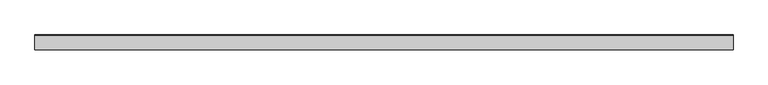
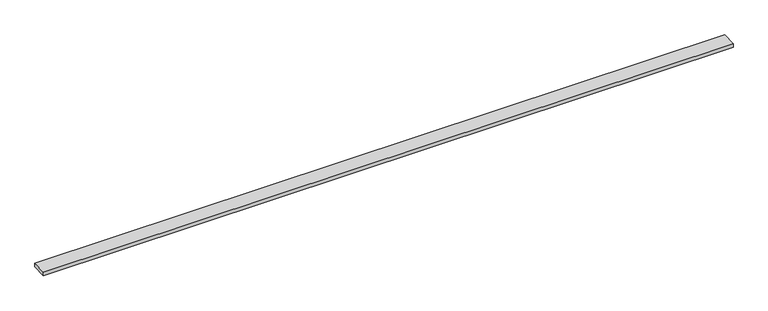
"""IFC4 building model written with IfcOpenShell, lengths in millimetres: proxy geometry, Inner panel:Inner panel:1:Inner panel:1 : Inner panel:Inner panel:300324:2:Inner panel:1:Inner panel:1 : Inner panel:Inner panel:300324:2 : Inner panel:Inner panel:1:Inner panel:1 : Inner panel:Inner panel:300324:300043:9 : Inner panel:Inner panel:1:Inner panel:1 : Inner panel:Inner panel:300324:2:Inner panel:1:Inner panel:1 : Inner panel:Inner panel:300324:2 : Inner panel:Inner panel:1:Inner panel:1 : Inner panel:Inner panel:300324:300043:308120."""

from ifc_helpers import new_model, si_unit, frame, origin, place, context, project, spatial, polyline, outline, extrude, source, transform, mapped, element, save


def generic_models_4ea8c6c7(model_context):
    return source(origin(), model_context, "Body", "SweptSolid", [
        extrude(outline(polyline([(0.0, -102.7190976), (0.0, 0.0), (4876.8, 0.0), (4876.8, -102.7190976), (0.0, -102.7190976)])), frame((596182.8367242, -536656.3145522, 10092.0375334), z_axis=(0.0, -0.04163054471218835, 0.9991330730923517), x_axis=(-1.0, 0.0, 0.0)), (0.0, 0.0, 1.0), 25.4),
    ])


if __name__ == "__main__":
    model = new_model("IFC4")
    model_context = context("Model", 3, world=origin())
    ifc_project = project(units=[si_unit("LENGTHUNIT", "METRE", prefix="MILLI")], contexts=[model_context])
    site = spatial("IfcSite", under=ifc_project)
    building = spatial("IfcBuilding", under=site)
    placement = place(None, origin())
    generic_models_shape = generic_models_4ea8c6c7(model_context)
    element("IfcBuildingElementProxy", 1, Name="Inner panel:Inner panel:1:Inner panel:1 : Inner panel:Inner panel:300324:2:Inner panel:1:Inner panel:1 : Inner panel:Inner panel:300324:2 : Inner panel:Inner panel:1:Inner panel:1 : Inner panel:Inner panel:300324:300043:9 : Inner panel:Inner panel:1:Inner panel:1 : Inner panel:Inner panel:300324:2:Inner panel:1:Inner panel:1 : Inner panel:Inner panel:300324:2 : Inner panel:Inner panel:1:Inner panel:1 : Inner panel:Inner panel:300324:300043:308120", ObjectType="Inner panel:Inner panel:1:Inner panel:1 : Inner panel:Inner panel:300324:2:Inner panel:1:Inner panel:1 : Inner panel:Inner panel:300324:2 : Inner panel:Inner panel:1:Inner panel:1 : Inner panel:Inner panel:300324:300043:9 : Inner panel:Inner panel:1:Inner panel:1 : Inner panel:Inner panel:300324:2:Inner panel:1:Inner panel:1 : Inner panel:Inner panel:300324:2 : Inner panel:Inner panel:1:Inner panel:1 : Inner panel:Inner panel:300324:300043:308120", at=placement, inside=building, context=model_context, shape_type="MappedRepresentation", body=[
        mapped(generic_models_shape, transform((0.0, 0.0, 0.0), x_axis=(1.0, 0.0, 0.0), y_axis=(0.0, 1.0, 0.0), z_axis=(0.0, 0.0, 1.0))),
    ])
    save(model, "model.ifc")

# Revit data of these elements
# Type "Inner panel:Inner panel:1:Inner panel:1 : Inner panel:Inner panel:300324:2:Inner panel:1:Inner panel:1 : Inner panel:Inner panel:300324:2 : Inner panel:Inner panel:1:Inner panel:1 : Inner panel:Inner panel:300324:300043:9 : Inner panel:Inner panel:1:Inner panel:1 : Inner panel:Inner panel:300324:2:Inner panel:1:Inner panel:1 : Inner panel:Inner panel:300324:2 : Inner panel:Inner panel:1:Inner panel:1 : Inner panel:Inner panel:300324:300043:308120"
#   NameOverride = "Inner panel:Inner panel:1:Inner panel:1 : Inner panel:Inner panel:300324:2:Inner panel:1:Inner panel:1 : Inner panel:Inner panel:300324:2 : Inner panel:Inner panel:1:Inner panel:1 : Inner panel:Inner panel:300324:300043:308120"
#   ObjectTypeOverride = "Inner panel:1:Inner panel:1 : Inner panel:Inner panel:300324:2 : Inner panel:Inner panel:1:Inner panel:1 : Inner panel:Inner panel:300324:300043"
#   Reference = "Inner panel"
#   Tag = "308120"
# Element 1 (IfcBuildingElementProxy, "Inner panel:Inner panel:1:Inner panel:1 : Inner panel:Inner panel:300324:2:Inner panel:1:Inner panel:1 : Inner panel:Inner panel:300324:2 : Inner panel:Inner panel:1:Inner panel:1 : Inner panel:Inner panel:300324:300043:9 : Inner panel:Inner panel:1:Inner panel:1 : Inner panel:Inner panel:300324:2:Inner panel:1:Inner panel:1 : Inner panel:Inner panel:300324:2 : Inner panel:Inner panel:1:Inner panel:1 : Inner panel:Inner panel:300324:300043:308120")
#   Materials on its faces: "1\" THERMAL SPACER @ PURLIN"
# Materials
#   "1\" THERMAL SPACER @ PURLIN": class "Unassigned", colour RGB 205 188 106, transparency 0, Cost = 0
